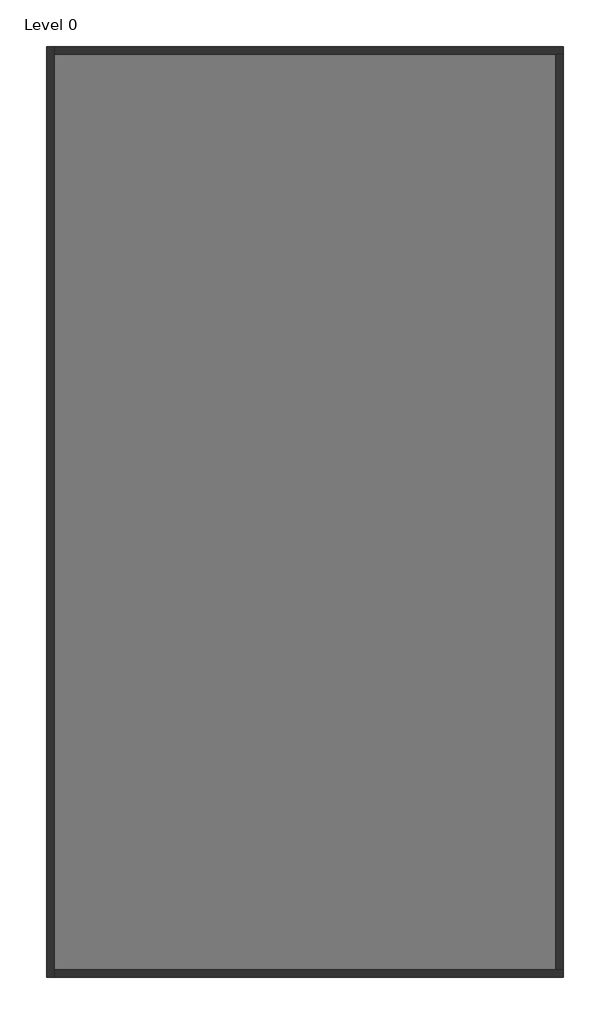
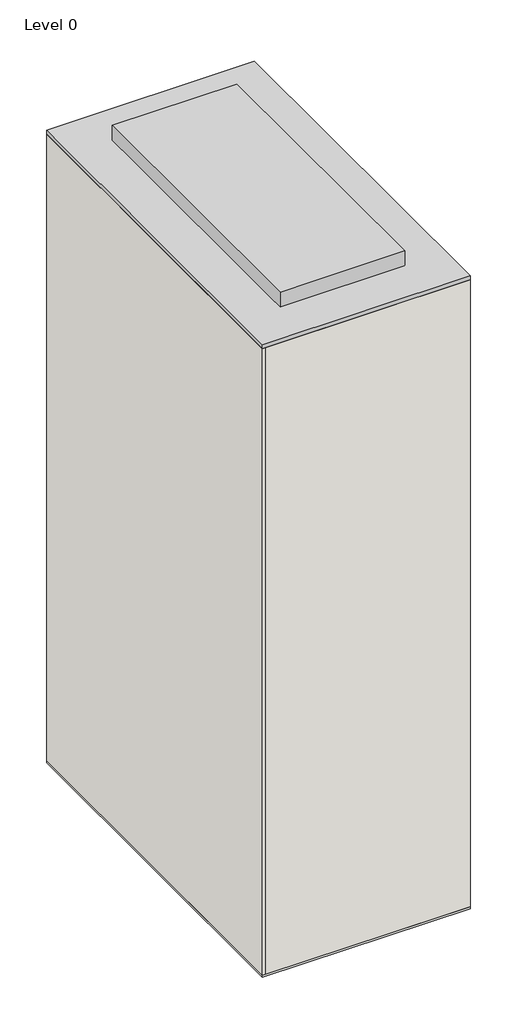
# One storey: 4 walls, 1 proxy, 1 slab.
"""IFC4 building model written with IfcOpenShell, lengths in millimetres."""

from ifc_helpers import new_model, si_unit, frame, origin, origin_with_axes, place, context, project, spatial, polyline, outline, extrude, faceted_brep, element, save

model = new_model("IFC4")

# Units and contexts
model_context = context("Model", 3, world=origin())
ifc_project = project(units=[si_unit("LENGTHUNIT", "METRE", prefix="MILLI")], contexts=[model_context])

# Site, building, storey
site = spatial("IfcSite", under=ifc_project)
building = spatial("IfcBuilding", under=site)
storey = spatial("IfcBuildingStorey", under=building, Name="Level 0", Elevation=100.0)

# Proxy
placement = place(None, origin())
element("IfcBuildingElementProxy", 1, Name="LowUrbanDensityBuilding : LowUrbanDensityBuilding", ObjectType="LowUrbanDensityBuilding : LowUrbanDensityBuilding", at=placement, inside=storey, context=model_context, shape_type="SweptSolid", body=[
    extrude(outline(polyline([(7325.2659446, 3676.2074539), (7325.2659446, -14323.7925461), (-2674.7340554, -14323.7925461), (-2674.7340554, 3676.2074539), (7325.2659446, 3676.2074539)])), origin_with_axes(), (0.0, 0.0, 1.0), 32200.0),
    extrude(outline(polyline([(5325.2659446, 1676.2074539), (5325.2659446, -12323.7925461), (-674.7340554, -12323.7925461), (-674.7340554, 1676.2074539), (5325.2659446, 1676.2074539)])), frame((0.0, 0.0, 32000.0), z_axis=(0.0, 0.0, 1.0), x_axis=(1.0, 0.0, 0.0)), (0.0, 0.0, 1.0), 949.8),
])

# Slab
element("IfcSlab", 2, ObjectType="Floor-Concrete_100Con", at=placement, inside=storey, context=model_context, shape_type="SweptSolid", body=[
    extrude(outline(polyline([(7325.2659446, 3676.2074539), (7325.2659446, -14323.7925461), (-2674.7340554, -14323.7925461), (-2674.7340554, 3676.2074539), (7325.2659446, 3676.2074539)])), origin_with_axes(), (0.0, 0.0, 1.0), 100.0),
])

# Walls
element("IfcWall", 3, ObjectType="Wall-Ext_25Rdr-100Blk-19P", at=placement, inside=storey, context=model_context, shape_type="Brep", body=[
    faceted_brep([(-2674.7340554, 3676.2074539, 100.0), (-2674.7340554, -14323.7925461, 100.0), (-2674.7340554, -14323.7925461, 32000.0), (-2674.7340554, 3676.2074539, 32000.0), (-2530.4340554, 3676.2074539, 100.0), (-2530.4340554, 3676.2074539, 32000.0), (-2530.4340554, 3531.9074539, 32000.0), (-2530.4340554, -14179.4925461, 32000.0), (-2530.4340554, -14323.7925461, 32000.0), (-2530.4340554, -14323.7925461, 100.0), (-2530.4340554, -14179.4925461, 100.0), (-2530.4340554, 3531.9074539, 100.0)], [[[0, 1, 2, 3]], [[4, 5, 6, 7, 8, 9, 10, 11]], [[1, 0, 4, 11, 10, 9]], [[3, 2, 8, 7, 6, 5]], [[2, 1, 9, 8]], [[0, 3, 5, 4]]]),
])
element("IfcWall", 4, ObjectType="Wall-Ext_25Rdr-100Blk-19P", at=placement, inside=storey, context=model_context, shape_type="Brep", body=[
    faceted_brep([(-2530.4340554, -14323.7925461, 100.0), (7325.2659446, -14323.7925461, 100.0), (7325.2659446, -14323.7925461, 32000.0), (-2530.4340554, -14323.7925461, 32000.0), (-2530.4340554, -14179.4925461, 100.0), (-2530.4340554, -14179.4925461, 32000.0), (7180.9659446, -14179.4925461, 32000.0), (7325.2659446, -14179.4925461, 32000.0), (7325.2659446, -14179.4925461, 100.0), (7180.9659446, -14179.4925461, 100.0)], [[[0, 1, 2, 3]], [[4, 5, 6, 7, 8, 9]], [[1, 0, 4, 9, 8]], [[3, 2, 7, 6, 5]], [[0, 3, 5, 4]], [[2, 1, 8, 7]]]),
])
element("IfcWall", 5, ObjectType="Wall-Ext_25Rdr-100Blk-19P", at=placement, inside=storey, context=model_context, shape_type="Brep", body=[
    faceted_brep([(7325.2659446, 3676.2074539, 100.0), (-2530.4340554, 3676.2074539, 100.0), (-2530.4340554, 3676.2074539, 32000.0), (7325.2659446, 3676.2074539, 32000.0), (7325.2659446, 3531.9074539, 100.0), (7325.2659446, 3531.9074539, 32000.0), (7180.9659446, 3531.9074539, 32000.0), (-2530.4340554, 3531.9074539, 32000.0), (-2530.4340554, 3531.9074539, 100.0), (7180.9659446, 3531.9074539, 100.0)], [[[0, 1, 2, 3]], [[4, 5, 6, 7, 8, 9]], [[1, 0, 4, 9, 8]], [[3, 2, 7, 6, 5]], [[2, 1, 8, 7]], [[0, 3, 5, 4]]]),
])
element("IfcWall", 6, ObjectType="Wall-Ext_25Rdr-100Blk-19P", at=placement, inside=storey, context=model_context, shape_type="SweptSolid", body=[
    extrude(outline(polyline([(7325.2659446, 3531.9074539), (7325.2659446, -14179.4925461), (7180.9659446, -14179.4925461), (7180.9659446, 3531.9074539), (7325.2659446, 3531.9074539)])), frame((0.0, 0.0, 100.0), z_axis=(0.0, 0.0, 1.0), x_axis=(1.0, 0.0, 0.0)), (0.0, 0.0, 1.0), 31900.0),
])

save(model, "model.ifc")

# Revit data of these elements
# Project information
#   Project Issue Date = "Issue Date"
#   Project Status = "Project Status"
#   Client Name = "Owner"
#   Project Address = "Enter address here"
#   Project Name = "Project Name"
#   Project Number = "Project Number"
# Type "Floor-Concrete_100Con"
#   Keynote = "E60/130"
#   Function = 0
#   Layers, outside or top first: 100 mm "Concrete" (function 1)
# Type "Wall-Ext_25Rdr-100Blk-19P"
#   Keynote = "F10"
#   Layers, outside or top first: 25.3 mm "Render, Beige, Smooth" (function 5); 100 mm "Concrete Masonry Units _Low Density" (function 1); 19 mm "Plaster" (function 5)
# Element 1 (IfcBuildingElementProxy, "LowUrbanDensityBuilding : LowUrbanDensityBuilding")
#   Phase Created = New Construction
#   Materials on its faces: "Default Form"
# Element 2 (IfcSlab, "Floor-Concrete_100Con")
#   Height Offset From Level = 0 mm
#   Phase Created = New Construction
#   Materials on its faces: "Concrete"
# Element 3 (IfcWall, "Wall-Ext_25Rdr-100Blk-19P")
#   Top Offset = 0 mm
#   Base Offset = 0 mm
#   wall height = 31900 mm
#   Phase Created = New Construction
#   Base Constraint = Level 0
#   Top Constraint = Level 8
#   Materials on its faces: "Render, Beige, Smooth", "Default Wall", "Plaster"
# Elements 4, 5, 6 (IfcWall, "Wall-Ext_25Rdr-100Blk-19P")
#   Top Offset = 0 mm
#   Base Offset = 0 mm
#   wall height = 31900 mm
#   Phase Created = New Construction
#   Base Constraint = Level 0
#   Top Constraint = Level 8
#   Materials on its faces: "Default Wall", "Render, Beige, Smooth", "Plaster"
# Materials
#   "Concrete": class "Concrete", colour RGB 120 120 120, transparency 0, Description = "Portland Cement Concrete", Cost = 0
#   "Render, Beige, Smooth": class "Generic", colour RGB 213 198 180, transparency 0, Description = "physical material", Cost = 0
#   "Concrete Masonry Units _Low Density": class "Masonry", colour RGB 181 181 181, transparency 0, Description = "Concrete masonry units", Cost = 0
#   "Plaster": class "Generic", colour RGB 249 249 249, transparency 0, Description = "Plaster", Cost = 0
#   "Default Form": class "Generic", colour RGB 185 189 196, transparency 0.5, Cost = 0
#   "Default Wall": class "Miscellaneous", colour RGB 128 128 128, transparency 0, Comments = "Rendering appearance not upgraded Rendering appearance not upgraded ", Cost = 0
